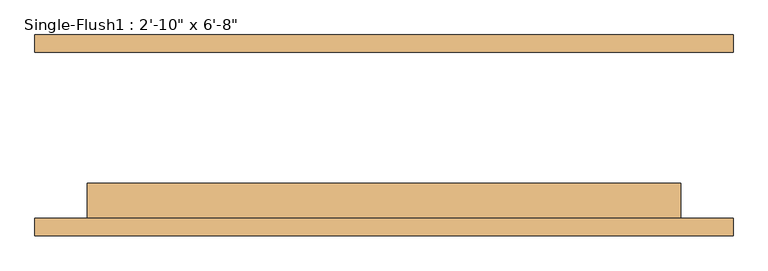
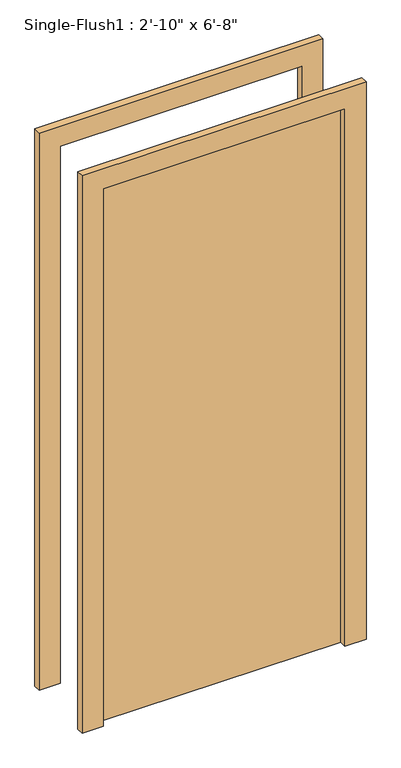
"""IFC4 building model written with IfcOpenShell, lengths in millimetres: door geometry."""

from ifc_helpers import new_model, si_unit, frame, origin, origin_with_axes, place, context, project, spatial, polyline, outline, extrude, source, transform, mapped, element, save


def door_8da58a41(model_context):
    return source(origin(), model_context, "Body", "SweptSolid", [
        extrude(outline(polyline([(2108.2, -508.0), (0.0, -508.0), (0.0, -431.8), (2032.0, -431.8), (2032.0, 431.8), (0.0, 431.8), (0.0, 508.0), (2108.2, 508.0), (2108.2, -508.0)])), frame((0.0, -146.05, 0.0), z_axis=(0.0, 1.0, 0.0), x_axis=(0.0, 0.0, 1.0)), (0.0, 0.0, 1.0), 25.4),
        extrude(outline(polyline([(2108.2, 508.0), (2108.2, -508.0), (0.0, -508.0), (0.0, -431.8), (2032.0, -431.8), (2032.0, 431.8), (0.0, 431.8), (0.0, 508.0), (2108.2, 508.0)])), frame((0.0, 120.65, 0.0), z_axis=(0.0, 1.0, 0.0), x_axis=(0.0, 0.0, 1.0)), (0.0, 0.0, 1.0), 25.4),
        extrude(outline(polyline([(431.8, -69.85), (431.8, -120.65), (-431.8, -120.65), (-431.8, -69.85), (431.8, -69.85)])), origin_with_axes(), (0.0, 0.0, 1.0), 2032.0),
    ])


if __name__ == "__main__":
    model = new_model("IFC4")
    model_context = context("Model", 3, world=origin())
    ifc_project = project(units=[si_unit("LENGTHUNIT", "METRE", prefix="MILLI")], contexts=[model_context])
    site = spatial("IfcSite", under=ifc_project)
    building = spatial("IfcBuilding", under=site)
    placement = place(None, origin())
    door_shape = door_8da58a41(model_context)
    element("IfcDoor", 1, ObjectType="Single-Flush1 : 2'-10\" x 6'-8\"", at=placement, inside=building, context=model_context, shape_type="MappedRepresentation", body=[
        mapped(door_shape, transform((0.0, 0.0, 0.0), x_axis=(1.0, 0.0, 0.0), y_axis=(0.0, 1.0, 0.0), z_axis=(0.0, 0.0, 1.0))),
    ])
    save(model, "model.ifc")

# Revit data of these elements
# Type "Single-Flush1 : 2'-10\" x 6'-8\""
#   Type Mark = "26"
#   Construction Type Id = "MDOOR"
#   Assembly Code = "C1020"
#   Analytic Construction = "Metal"
#   Thickness = 0' - 2"
#   Heat Transfer Coefficient (U) = 3.7021 W/(m²·K)
#   Height = 6' - 8"
#   Trim Projection Ext = 0' - 1"
#   Trim Projection Int = 0' - 1"
#   Trim Width = 0' - 3"
#   Width = 2' - 10"
#   Door Material = Door - Panel
#   Frame Material = Door - Frame
#   Visual Light Transmittance = 0
#   Solar Heat Gain Coefficient = 0
#   Function = (empty or 0)
#   Wall Closure = (empty or 0)
# Element 1 (IfcDoor, "Single-Flush1 : 2'-10\" x 6'-8\"")
#   Materials on its faces: "Door - Frame", "Door - Panel"
# Materials
#   "Door - Panel": class "Wood", colour RGB 210 159 95, transparency 0, Cost = 0
#   "Door - Frame": class "Miscellaneous", colour RGB 118 70 51, transparency 0, Cost = 0
